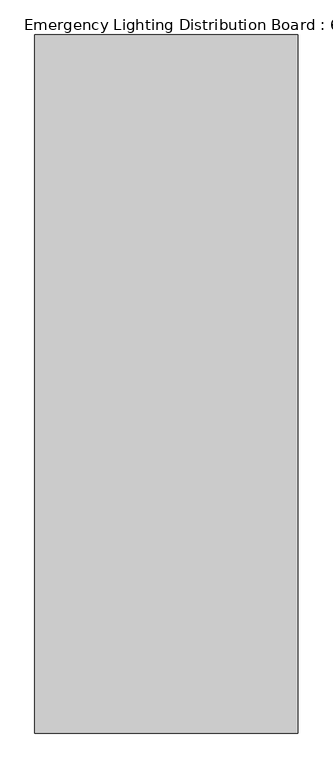
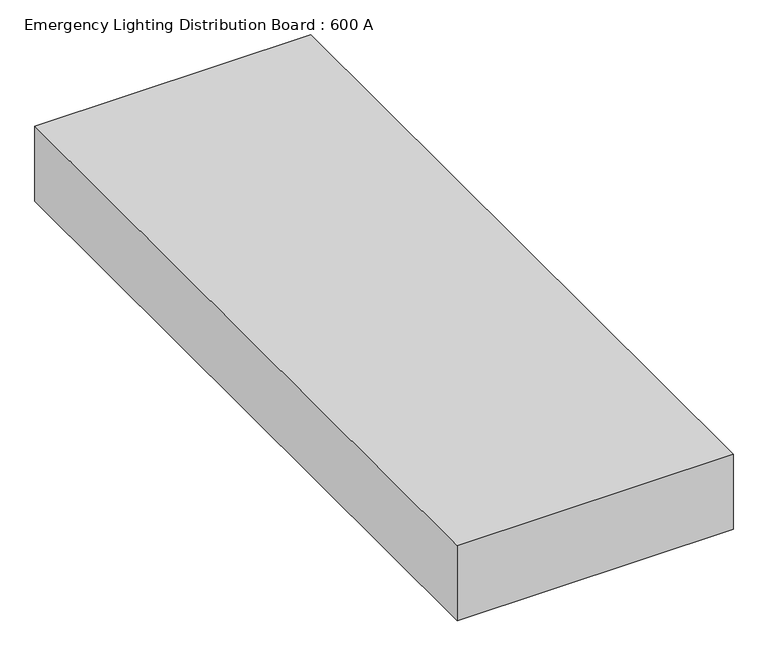
"""IFC4 building model written with IfcOpenShell, lengths in millimetres: proxy geometry, Emergency Lighting Distribution Board : 600 A."""

from ifc_helpers import new_model, si_unit, origin, origin_with_axes, place, context, project, spatial, polyline, outline, extrude, source, transform, mapped, element, save


def emergency_lighting_distribution_board_600_a_cf68ca70(model_context):
    return source(origin(), model_context, "Body", "SweptSolid", [
        extrude(outline(polyline([(254.0, -1346.2), (-254.0, -1346.2), (-254.0, 0.0), (254.0, 0.0), (254.0, -1346.2)])), origin_with_axes(), (0.0, 0.0, 1.0), 146.1),
    ])


if __name__ == "__main__":
    model = new_model("IFC4")
    model_context = context("Model", 3, world=origin())
    ifc_project = project(units=[si_unit("LENGTHUNIT", "METRE", prefix="MILLI")], contexts=[model_context])
    site = spatial("IfcSite", under=ifc_project)
    building = spatial("IfcBuilding", under=site)
    placement = place(None, origin())
    emergency_lighting_distribution_board_600_a_shape = emergency_lighting_distribution_board_600_a_cf68ca70(model_context)
    element("IfcBuildingElementProxy", 1, Name="Emergency Lighting Distribution Board : 600 A", ObjectType="Emergency Lighting Distribution Board : 600 A", at=placement, inside=building, context=model_context, shape_type="MappedRepresentation", body=[
        mapped(emergency_lighting_distribution_board_600_a_shape, transform((0.0, 0.0, 0.0), x_axis=(1.0, 0.0, 0.0), y_axis=(0.0, 1.0, 0.0), z_axis=(0.0, 0.0, 1.0))),
    ])
    save(model, "model.ifc")

# Revit data of these elements
# Type "Emergency Lighting Distribution Board : 600 A"
#   Type Mark = "Emergency Lighting Distribution Board"
#   Classification.OmniClass.21.Number = "21-04 50 40 50"
#   Classification.OmniClass.21.Description = "Lighting Fixtures"
#   Classification.UniFormat.II.Description = "Lighting Fixtures"
#   Classification.OmniClass.23.Number = "23-35 31 13"
#   Classification.OmniClass.23.Description = "Distribution Panel Boards"
#   Classification.UniFormat.II.Number = "D5040.50"
#   COBie.Type.CreatedBy = "info@mma.ie"
#   COBie.Type.CreatedOn = "2017-07-25T10:15:16"
#   COBie.Type.Name = "Emergency Lighting Distribution Board"
#   COBie.Type.Category = "23-35 31 13 : Distribution Panel Boards"
#   COBie.Type.Description = "Emergency Lighting Distribution Board_600 A"
#   COBie.Type.AssetType = "Fixed"
#   COBie.Type.Manufacturer = ""
#   COBie.Type.ModelNumber = ""
#   Wattage = "400"
#   Voltage = "600"
#   built-in parameter 1140081 [instance default] = "Recessed"
#   Keynote = "26 26 00.A"
#   built-in parameter 1140083 [instance default] = "Type 1"
#   COBie.Type.ReplacementCost = 0
#   Width = 508 mm
#   built-in parameter 1140082 [instance default] = 100 (stored number, unit not read)
#   built-in parameter 1140140 [instance default] = 600 (stored number, unit not read)
#   Height [instance default] = 1346.2 mm
#   ELDB Width = 508 mm
#   ELDB Height = 1346.2 mm
#   ELDB Depth = 146.1 mm
#   Depth = 146.1 mm
#   Default Elevation = 1200 mm
#   Ballast Wattage = 400 W
#   Ballast Voltage = 600 V
#   42 Circuit Height = 1879.6 mm
#   30 Circuit Height = 1651 mm
#   24 Circuit Height = 1346.2 mm
#   12 Circuit Height = 1346.2 mm
#   COBie.Type = yes
#   built-in parameter 1140142 [instance default] = -1
#   built-in parameter 1140079 [instance default] = 12
#   built-in parameter 1155100 [instance default] = -1
#   Load Classification = Other
